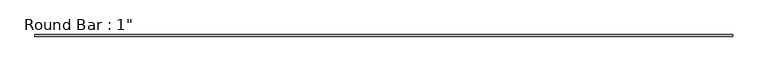
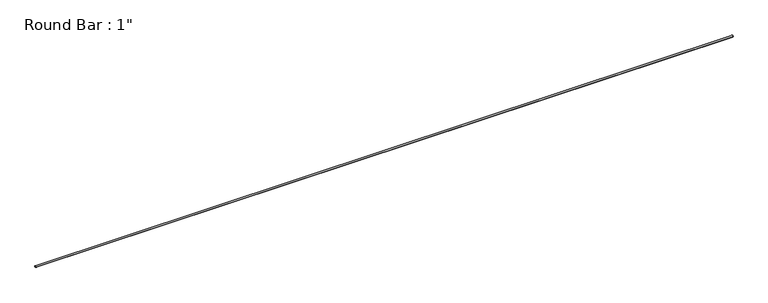
"""IFC4 building model written with IfcOpenShell, lengths in millimetres: member geometry."""

from ifc_helpers import new_model, si_unit, point, frame, origin, origin_2d, place, context, project, spatial, circle_curve, trimmed, segment, composite_curve, outline, extrude, source, transform, mapped, element, save


def member_e1aa61fe(model_context):
    return source(origin(), model_context, "Body", "SweptSolid", [
        extrude(outline(composite_curve([segment(trimmed(circle_curve(origin_2d(), 12.7), [point((-12.7, 0.0))], [point((12.7, 0.0))], False, "CARTESIAN"), True, "CONTINUOUS"), segment(trimmed(circle_curve(origin_2d(), 12.7), [point((12.7, 0.0))], [point((-12.7, 0.0))], False, "CARTESIAN"), True, "CONTINUOUS")], self_intersect=False)), frame((-5425.0253699, 0.0, 0.0), z_axis=(1.0, 0.0, 0.0), x_axis=(0.0, 1.0, 0.0)), (0.0, 0.0, 1.0), 10850.0507398),
    ])


if __name__ == "__main__":
    model = new_model("IFC4")
    model_context = context("Model", 3, world=origin())
    ifc_project = project(units=[si_unit("LENGTHUNIT", "METRE", prefix="MILLI")], contexts=[model_context])
    site = spatial("IfcSite", under=ifc_project)
    building = spatial("IfcBuilding", under=site)
    placement = place(None, origin())
    member_shape = member_e1aa61fe(model_context)
    element("IfcMember", 1, ObjectType="Round Bar : 1\"", at=placement, inside=building, context=model_context, shape_type="MappedRepresentation", body=[
        mapped(member_shape, transform((0.0, 0.0, 0.0), x_axis=(1.0, 0.0, 0.0), y_axis=(0.0, 1.0, 0.0), z_axis=(0.0, 0.0, 1.0))),
    ])
    save(model, "model.ifc")

# Revit data of these elements
# Type "Round Bar : 1\""
#   Assembly Code = "B10"
#   W = 0
#   Start Extension Calculation [instance default] = 10' - 0"
#   Start Extension [instance default] = -0' - 0 1/2"
#   End Extension Calculation [instance default] = 10' - 0"
#   End Extension [instance default] = -0' - 0 1/2"
#   Length [instance default] = 5' - 0"
#   d = 0' - 1"
#   A = 0 SF
#   Structural Material [instance default] = Metal - Steel - ASTM A36
# Element 1 (IfcMember, "Round Bar : 1\"")
#   Materials on its faces: "Metal - Steel - ASTM A36"
# Materials
#   "Metal - Steel - ASTM A36": class "Metal", colour RGB 199 199 199, transparency 0
